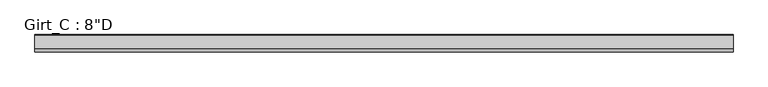
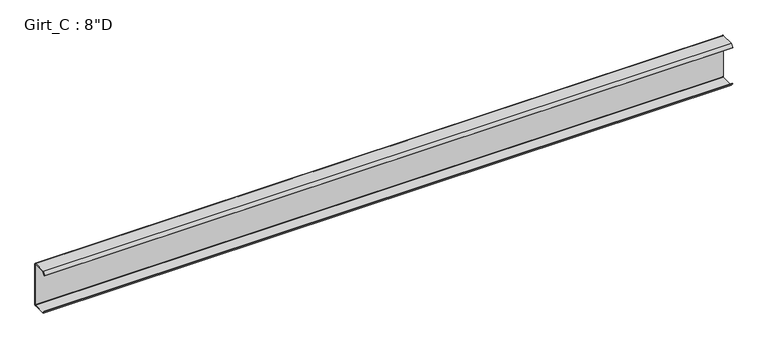
"""IFC4 building model written with IfcOpenShell, lengths in millimetres: beam geometry."""

from ifc_helpers import new_model, si_unit, point, frame, frame_2d, origin, place, context, project, spatial, polyline, circle_curve, trimmed, segment, composite_curve, outline, extrude, source, transform, mapped, element, save


def beam_8deb2c59(model_context):
    return source(origin(), model_context, "Body", "SweptSolid", [
        extrude(outline(composite_curve([segment(polyline([(-63.5, 101.6), (-3.3734375, 101.6)]), True, "CONTINUOUS"), segment(trimmed(circle_curve(frame_2d((-3.3734375, 96.8375)), 4.7625), [point((-3.3734375, 101.6))], [point((1.3890625, 96.8375))], False, "CARTESIAN"), True, "CONTINUOUS"), segment(polyline([(1.3890625, 96.8375), (1.3890625, -96.8375)]), True, "CONTINUOUS"), segment(trimmed(circle_curve(frame_2d((-3.3734375, -96.8375)), 4.7625), [point((1.3890625, -96.8375))], [point((-3.3734375, -101.6))], False, "CARTESIAN"), True, "CONTINUOUS"), segment(polyline([(-3.3734375, -101.6), (-63.5, -101.6), (-75.745104, -87.0068534), (-73.6169367, -85.221109), (-62.204539, -98.821875), (-3.2694106, -98.821875)]), True, "CONTINUOUS"), segment(trimmed(circle_curve(frame_2d((-3.3748024, -96.8389339)), 1.9857399), [point((-3.2694106, -98.821875))], [point((-1.3890625, -96.8389339))], True, "CARTESIAN"), True, "CONTINUOUS"), segment(polyline([(-1.3890625, -96.8389339), (-1.3890625, 96.8381931)]), True, "CONTINUOUS"), segment(trimmed(circle_curve(frame_2d((-3.3741066, 96.8381931)), 1.9850441), [point((-1.3890625, 96.8381931))], [point((-3.3005807, 98.821875))], True, "CARTESIAN"), True, "CONTINUOUS"), segment(polyline([(-3.3005807, 98.821875), (-62.204539, 98.821875), (-73.6169367, 85.221109), (-75.745104, 87.0068534), (-63.5, 101.6)]), True, "CONTINUOUS")], self_intersect=False)), frame((-1562.1, 0.0, 0.0), z_axis=(1.0, 0.0, 0.0), x_axis=(0.0, 1.0, 0.0)), (0.0, 0.0, 1.0), 3124.2),
    ])


if __name__ == "__main__":
    model = new_model("IFC4")
    model_context = context("Model", 3, world=origin())
    ifc_project = project(units=[si_unit("LENGTHUNIT", "METRE", prefix="MILLI")], contexts=[model_context])
    site = spatial("IfcSite", under=ifc_project)
    building = spatial("IfcBuilding", under=site)
    placement = place(None, origin())
    beam_shape = beam_8deb2c59(model_context)
    element("IfcBeam", 1, ObjectType="Girt_C : 8\"D", at=placement, inside=building, context=model_context, shape_type="MappedRepresentation", body=[
        mapped(beam_shape, transform((0.0, 0.0, 0.0), x_axis=(1.0, 0.0, 0.0), y_axis=(0.0, 1.0, 0.0), z_axis=(0.0, 0.0, 1.0))),
    ])
    save(model, "model.ifc")

# Revit data of these elements
# Type "Girt_C : 8\"D"
#   Web_Thickness = 0' - 0 7/64"
#   Length [instance default] = 10' - 0"
#   Leg_1 = 0' - 2 1/2"
#   Height = 0' - 8"
#   Structural Material [instance default] = none
# Element 1 (IfcBeam, "Girt_C : 8\"D")
#   Structural Material = Steel
#   Materials on its faces: "Steel"
# Materials
#   "Steel": class "Metal", colour RGB 118 118 114, transparency 0, Description = "Steel, mill finish", Cost = 0
